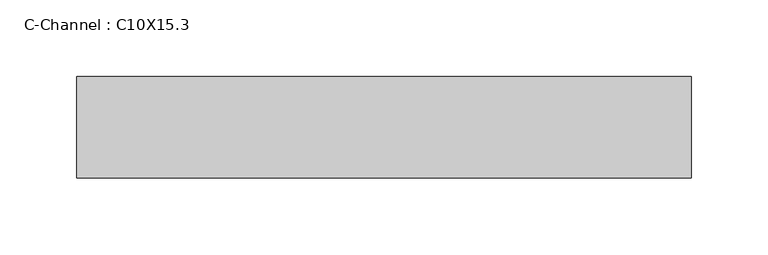
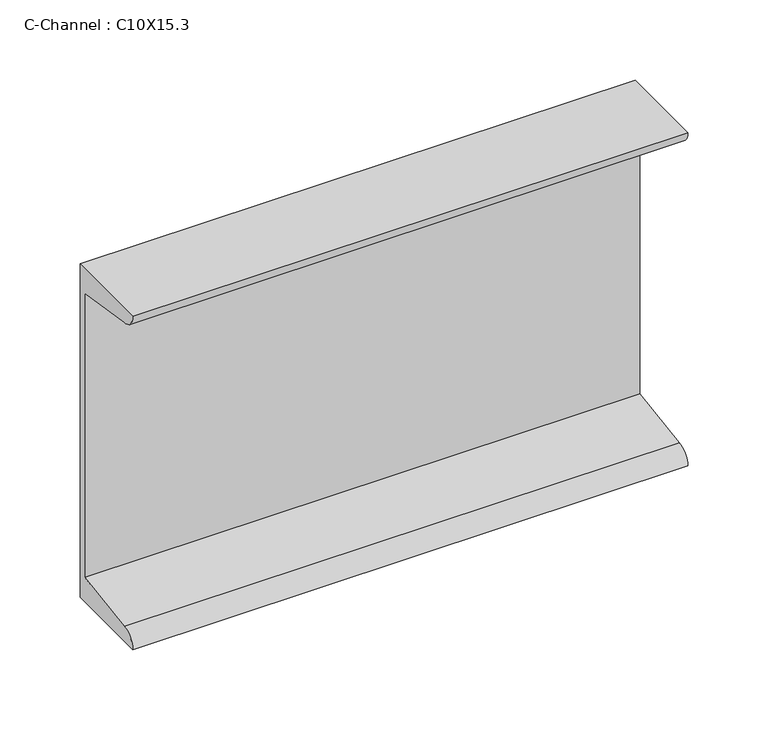
"""IFC4 building model written with IfcOpenShell, lengths in millimetres: beam geometry, C-Channel : C10X15.3."""

from ifc_helpers import new_model, si_unit, point, frame, frame_2d, origin, place, context, project, spatial, polyline, circle_curve, trimmed, segment, composite_curve, outline, extrude, source, transform, mapped, element, save


def c_channel_c10x15_3_d4be02f2(model_context):
    return source(origin(), model_context, "Body", "SweptSolid", [
        extrude(outline(composite_curve([segment(polyline([(16.1036, 127.0), (16.1036, -127.0), (-49.9364, -127.0)]), True, "CONTINUOUS"), segment(trimmed(circle_curve(frame_2d((-38.862, -127.0)), 11.0744), [point((-49.9364, -127.0))], [point((-38.862, -115.9256))], False, "CARTESIAN"), True, "CONTINUOUS"), segment(polyline([(-38.862, -115.9256), (10.0076, -108.1854158), (10.0076, 108.1854158), (-38.862, 115.9256)]), True, "CONTINUOUS"), segment(trimmed(circle_curve(frame_2d((-38.862, 127.0)), 11.0744), [point((-38.862, 115.9256))], [point((-49.9364, 127.0))], False, "CARTESIAN"), True, "CONTINUOUS"), segment(polyline([(-49.9364, 127.0), (16.1036, 127.0)]), True, "CONTINUOUS")], self_intersect=False)), frame((-127.0, 0.0, 0.0), z_axis=(1.0, 0.0, 0.0), x_axis=(0.0, 1.0, 0.0)), (0.0, 0.0, 1.0), 400.05),
    ])


if __name__ == "__main__":
    model = new_model("IFC4")
    model_context = context("Model", 3, world=origin())
    ifc_project = project(units=[si_unit("LENGTHUNIT", "METRE", prefix="MILLI")], contexts=[model_context])
    site = spatial("IfcSite", under=ifc_project)
    building = spatial("IfcBuilding", under=site)
    placement = place(None, origin())
    c_channel_c10x15_3_shape = c_channel_c10x15_3_d4be02f2(model_context)
    element("IfcBeam", 1, ObjectType="C-Channel : C10X15.3", at=placement, inside=building, context=model_context, shape_type="MappedRepresentation", body=[
        mapped(c_channel_c10x15_3_shape, transform((0.0, 0.0, 0.0), x_axis=(1.0, 0.0, 0.0), y_axis=(0.0, 1.0, 0.0), z_axis=(0.0, 0.0, 1.0))),
    ])
    save(model, "model.ifc")

# Revit data of these elements
# Type "C-Channel : C10X15.3"
#   Assembly Code = "B10"
#   W = 15.3
#   Length [instance default] = 5' - 0"
#   bf = 0' - 2.6"
#   d = 0' - 10"
#   tf = 0' - 0.436"
#   tw = 0' - 0.24"
#   x = 0' - 0.634"
#   A = 0.0311111 SF
#   Structural Material [instance default] = Steel ASTM A36
# Element 1 (IfcBeam, "C-Channel : C10X15.3")
#   Structural Material = Steel ASTM A992
#   Materials on its faces: "Steel ASTM A992"
# Materials
#   "Steel ASTM A36": class "Metal", colour RGB 199 199 199, transparency 0, Description = "Structural steel, ASTM A36 Grade B, mill finish", Cost = 0
#   "Steel ASTM A992": class "Metal", colour RGB 199 199 199, transparency 0, Description = "Structural steel 50ksi", Cost = 0
